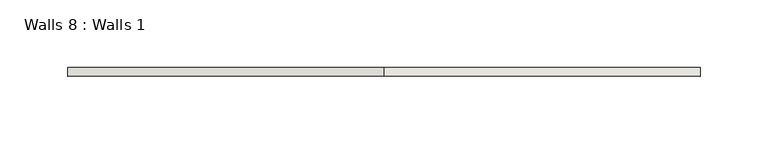
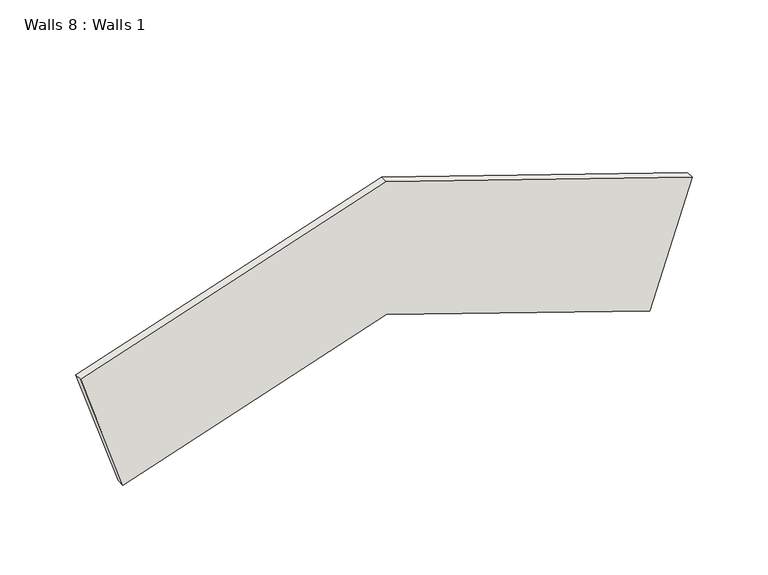
"""IFC4 building model written with IfcOpenShell, lengths in millimetres: wall geometry, Walls 8 : Walls 1."""

import ifcopenshell
import ifcopenshell.guid

model = None  # the IFC model being written
_history = None  # IfcOwnerHistory: only IFC2X3 demands one
_inside = {}  # id of a spatial element -> (the spatial element, [elements in it])
_under = {}  # id of a project, library or spatial element -> (it, [spatial elements below it])
_declared = {}  # id of a project -> (the project, [libraries it declares])
_typed = {}  # id of a type object -> (the type object, [elements of that type])
_made_of = {}  # id of a material, layer set ... -> (it, [elements and type objects made of it])


def new_model(schema):
    """Start an empty IFC model of exactly this schema.

    Asked for "IFC4X3", IfcOpenShell would pick the latest addendum, in which some entities
    have other attributes; the version numbers below select the first issue.
    IFC2X3 requires an IfcOwnerHistory on every rooted entity: one is made here for all.
    """
    global model, _history
    if schema == "IFC4X3":
        model = ifcopenshell.file(schema_version=(4, 3, 0, 0))
    else:
        model = ifcopenshell.file(schema=schema)
    _inside.clear()
    _under.clear()
    _declared.clear()
    _typed.clear()
    _made_of.clear()
    _history = None
    if model.schema == "IFC2X3":
        org = make("IfcOrganization", Name="unknown")
        user = make(
            "IfcPersonAndOrganization",
            ThePerson=make("IfcPerson", FamilyName="unknown"),
            TheOrganization=org,
        )
        app = make(
            "IfcApplication",
            ApplicationDeveloper=org,
            Version="unknown",
            ApplicationFullName="unknown",
            ApplicationIdentifier="unknown",
        )
        _history = make(
            "IfcOwnerHistory",
            OwningUser=user,
            OwningApplication=app,
            ChangeAction="ADDED",
            CreationDate=0,
        )
    return model


def make(cls, **values):
    """One entity of the class cls with the attributes given. An attribute that is None is left unset."""
    return model.create_entity(
        cls, **{name: value for name, value in values.items() if value is not None}
    )


def rooted(cls, **values):
    """An entity with a GlobalId (a new one), such as an element, a storey or a relation."""
    return make(cls, GlobalId=ifcopenshell.guid.new(), OwnerHistory=_history, **values)


def si_unit(unit_type, name, prefix=None):
    """IfcSIUnit, for example si_unit("LENGTHUNIT", "METRE", prefix="MILLI")."""
    return make("IfcSIUnit", UnitType=unit_type, Prefix=prefix, Name=name)


def assignment(units):
    """IfcUnitAssignment: the units of a project."""
    return None if units is None else make("IfcUnitAssignment", Units=units)


def point(xyz):
    """IfcCartesianPoint."""
    return None if xyz is None else make("IfcCartesianPoint", Coordinates=xyz)


def direction(xyz):
    """IfcDirection."""
    return None if xyz is None else make("IfcDirection", DirectionRatios=xyz)


def frame(location, z_axis=None, x_axis=None):
    """IfcAxis2Placement3D, a coordinate frame: its origin and axes. An axis left out is left unset."""
    return make(
        "IfcAxis2Placement3D",
        Location=point(location),
        Axis=direction(z_axis),
        RefDirection=direction(x_axis),
    )


def origin():
    """The frame at (0, 0, 0) with its axes left unset."""
    return frame((0.0, 0.0, 0.0))


def place(relative_to, where):
    """IfcLocalPlacement: puts the frame where relative to a parent placement (None: the world)."""
    return make(
        "IfcLocalPlacement", PlacementRelTo=relative_to, RelativePlacement=where
    )


def context(
    kind, dimensions, precision=None, world=None, true_north=None, identifier=None
):
    """IfcGeometricRepresentationContext, for example the 3D "Model" context."""
    return make(
        "IfcGeometricRepresentationContext",
        ContextIdentifier=identifier,
        ContextType=kind,
        CoordinateSpaceDimension=dimensions,
        Precision=precision,
        WorldCoordinateSystem=world,
        TrueNorth=true_north,
    )


def project(units=None, contexts=None):
    """IfcProject with its units and contexts."""
    return rooted(
        "IfcProject",
        Name="project",
        RepresentationContexts=contexts,
        UnitsInContext=assignment(units),
    )


def spatial(cls, under=None, at=None, **own):
    """A site, building, storey or space (cls), placed at a placement, below another one or the project."""
    s = rooted(cls, ObjectPlacement=at, **own)
    if under is not None:
        _under.setdefault(under.id(), (under, []))[1].append(s)
    return s


def polyline(points):
    """IfcPolyline through the points."""
    return make("IfcPolyline", Points=[point(p) for p in points])


def outline(outer, holes=None, kind="AREA"):
    """IfcArbitraryClosedProfileDef: a profile drawn as a closed curve; with holes, ...WithVoids."""
    if holes is None:
        return make("IfcArbitraryClosedProfileDef", ProfileType=kind, OuterCurve=outer)
    return make(
        "IfcArbitraryProfileDefWithVoids",
        ProfileType=kind,
        OuterCurve=outer,
        InnerCurves=holes,
    )


def extrude(swept, where, along, depth):
    """IfcExtrudedAreaSolid: the profile swept, set in the frame where, extruded along a direction by depth."""
    return make(
        "IfcExtrudedAreaSolid",
        SweptArea=swept,
        Position=where,
        ExtrudedDirection=direction(along),
        Depth=depth,
    )


def shape(context_of_items, identifier, shape_type, items):
    """IfcShapeRepresentation: the items that make up one representation, for example the "Body"."""
    return make(
        "IfcShapeRepresentation",
        ContextOfItems=context_of_items,
        RepresentationIdentifier=identifier,
        RepresentationType=shape_type,
        Items=items,
    )


def source(mapping_origin, context_of_items, identifier, shape_type, items):
    """IfcRepresentationMap: a shape defined once, which mapped items show again and again."""
    return make(
        "IfcRepresentationMap",
        MappingOrigin=mapping_origin,
        MappedRepresentation=shape(context_of_items, identifier, shape_type, items),
    )


def transform(
    local_origin,
    x_axis=None,
    y_axis=None,
    z_axis=None,
    scale=None,
    scale2=None,
    scale3=None,
    uniform=True,
):
    """IfcCartesianTransformationOperator3D, or its non-uniform kind. x_axis, y_axis, z_axis: its Axis1, 2, 3."""
    if uniform:
        return make(
            "IfcCartesianTransformationOperator3D",
            Axis1=direction(x_axis),
            Axis2=direction(y_axis),
            LocalOrigin=point(local_origin),
            Scale=scale,
            Axis3=direction(z_axis),
        )
    return make(
        "IfcCartesianTransformationOperator3DnonUniform",
        Axis1=direction(x_axis),
        Axis2=direction(y_axis),
        LocalOrigin=point(local_origin),
        Scale=scale,
        Axis3=direction(z_axis),
        Scale2=scale2,
        Scale3=scale3,
    )


def mapped(mapping_source, mapping_target):
    """IfcMappedItem: shows the shape of a source again, moved by a transform."""
    return make(
        "IfcMappedItem", MappingSource=mapping_source, MappingTarget=mapping_target
    )


def made_of(thing, what):
    """Note that an element or type object is made of a material, layer set ...; save() writes the relation."""
    if what is not None:
        _made_of.setdefault(what.id(), (what, []))[1].append(thing)
    return thing


def element(
    cls,
    number,
    at=None,
    inside=None,
    cuts=None,
    type_object=None,
    material=None,
    context=None,
    identifier="Body",
    shape_type=None,
    held_by="IfcProductDefinitionShape",
    body=None,
    shapes=None,
    **own,
):
    """One element of the class cls, such as IfcWall. Its Tag is "e" and its number.

    at: its placement. inside: the storey or other place that contains it. cuts: it is an
    opening in that element (IfcRelVoidsElement). A single representation is given by context,
    identifier, shape_type and body (its items); several are given by shapes. held_by: the class
    of the entity that holds the representations. save() writes the other relations.
    """
    e = rooted(cls, Tag="e%d" % number, ObjectPlacement=at, **own)
    if body is not None:
        shapes = [shape(context, identifier, shape_type, body)]
    if shapes is not None:
        e.Representation = make(held_by, Representations=shapes)
    if inside is not None:
        _inside.setdefault(inside.id(), (inside, []))[1].append(e)
    if cuts is not None:
        rooted(
            "IfcRelVoidsElement", RelatingBuildingElement=cuts, RelatedOpeningElement=e
        )
    if type_object is not None:
        _typed.setdefault(type_object.id(), (type_object, []))[1].append(e)
    return made_of(e, material)


def aggregate(whole, parts):
    """IfcRelAggregates: a whole, such as a stair, and the parts it consists of."""
    return rooted("IfcRelAggregates", RelatingObject=whole, RelatedObjects=parts)


def save(model, path):
    """Write the relations noted so far, then the file.

    IfcRelAggregates (storeys below a building ...), IfcRelContainedInSpatialStructure (elements
    in a storey), IfcRelDefinesByType, IfcRelAssociatesMaterial and IfcRelDeclares: one each for
    every whole, place, type object, material and project.
    """
    for whole, parts in _under.values():
        aggregate(whole, parts)
    for where, things in _inside.values():
        rooted(
            "IfcRelContainedInSpatialStructure",
            RelatedElements=things,
            RelatingStructure=where,
        )
    for kind, things in _typed.values():
        rooted("IfcRelDefinesByType", RelatedObjects=things, RelatingType=kind)
    for what, things in _made_of.values():
        rooted("IfcRelAssociatesMaterial", RelatedObjects=things, RelatingMaterial=what)
    for by, libraries in _declared.values():
        rooted("IfcRelDeclares", RelatingContext=by, RelatedDefinitions=libraries)
    model.write(path)


def walls_8_walls_1_fac39cad(model_context):
    return source(origin(), model_context, "Body", "SweptSolid", [
        extrude(outline(polyline([(5458.0690223, 21244.0906427), (5525.2438111, 21444.7370052), (5458.0690223, 21645.3833677), (5554.4130034, 21677.6385579), (5632.3865706, 21444.7370052), (5554.4130034, 21211.8354525), (5458.0690223, 21244.0906427)])), frame((0.0, -976.6384634, 0.0), z_axis=(0.0, 1.0, 0.0), x_axis=(0.0, 0.0, 1.0)), (0.0, 0.0, 1.0), 6.35),
    ])


if __name__ == "__main__":
    model = new_model("IFC4")
    model_context = context("Model", 3, world=origin())
    ifc_project = project(units=[si_unit("LENGTHUNIT", "METRE", prefix="MILLI")], contexts=[model_context])
    site = spatial("IfcSite", under=ifc_project)
    building = spatial("IfcBuilding", under=site)
    placement = place(None, origin())
    walls_8_walls_1_shape = walls_8_walls_1_fac39cad(model_context)
    element("IfcWall", 1, ObjectType="Walls 8 : Walls 1", at=placement, inside=building, context=model_context, shape_type="MappedRepresentation", body=[
        mapped(walls_8_walls_1_shape, transform((0.0, 0.0, 0.0), x_axis=(1.0, 0.0, 0.0), y_axis=(0.0, 1.0, 0.0), z_axis=(0.0, 0.0, 1.0))),
    ])
    save(model, "model.ifc")

# Revit data of these elements
# Element 1 (IfcWall, "Walls 8 : Walls 1")
#   Materials on its faces: "1/4\" STEEL GUSSET PLATE - (RAW STEEL)"
# Materials
#   "1/4\" STEEL GUSSET PLATE - (RAW STEEL)": class "Metal", colour RGB 189 187 185, transparency 0, Description = "Structural steel 50ksi", Cost = 0
